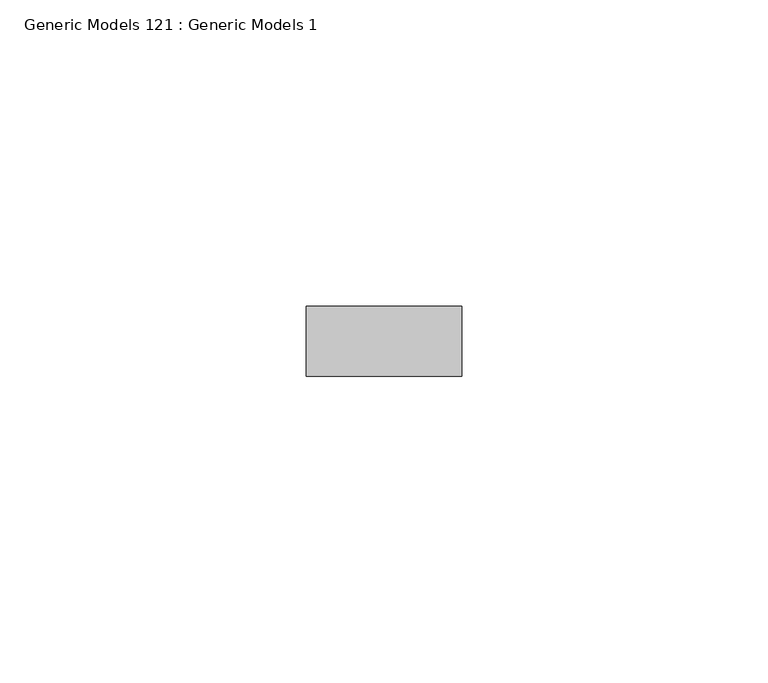
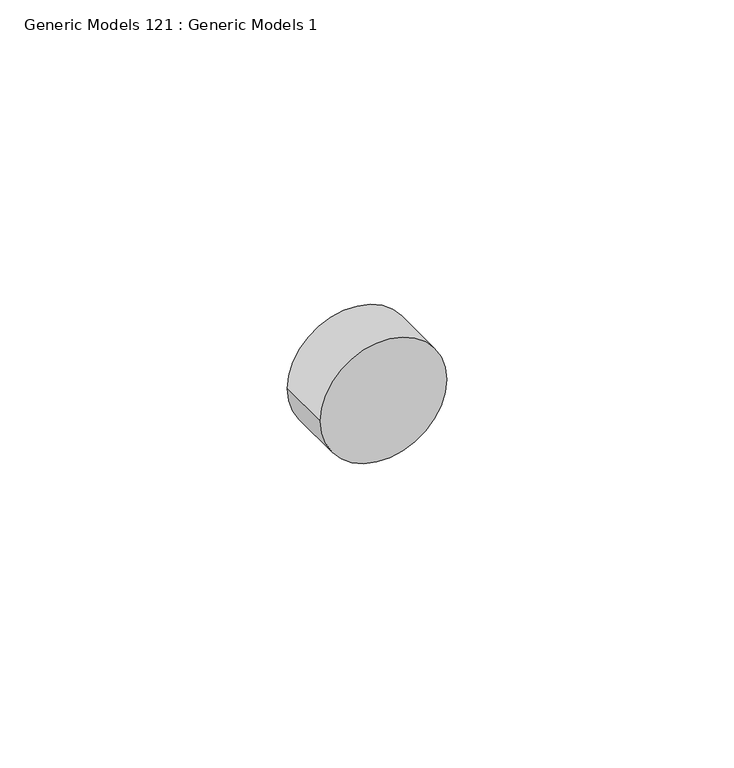
"""IFC4 building model written with IfcOpenShell, lengths in millimetres: proxy geometry, Generic Models 121 : Generic Models 1."""

from ifc_helpers import new_model, si_unit, point, frame, frame_2d, origin, place, context, project, spatial, circle_curve, trimmed, segment, composite_curve, outline, extrude, source, transform, mapped, element, save


def generic_models_121_generic_models_1_0d526897(model_context):
    return source(origin(), model_context, "Body", "SweptSolid", [
        extrude(outline(composite_curve([segment(trimmed(circle_curve(frame_2d((38203.4419837, 7407.5828124)), 12.7), [point((38203.4419837, 7394.8828124))], [point((38203.4419837, 7420.2828124))], False, "CARTESIAN"), True, "CONTINUOUS"), segment(trimmed(circle_curve(frame_2d((38203.4419837, 7407.5828124)), 12.7), [point((38203.4419837, 7420.2828124))], [point((38203.4419837, 7394.8828124))], False, "CARTESIAN"), True, "CONTINUOUS")], self_intersect=False)), frame((0.0, 1836.9202358, 0.0), z_axis=(0.0, 1.0, 0.0), x_axis=(0.0, 0.0, 1.0)), (0.0, 0.0, 1.0), 11.4464372),
    ])


if __name__ == "__main__":
    model = new_model("IFC4")
    model_context = context("Model", 3, world=origin())
    ifc_project = project(units=[si_unit("LENGTHUNIT", "METRE", prefix="MILLI")], contexts=[model_context])
    site = spatial("IfcSite", under=ifc_project)
    building = spatial("IfcBuilding", under=site)
    placement = place(None, origin())
    generic_models_121_generic_models_1_shape = generic_models_121_generic_models_1_0d526897(model_context)
    element("IfcBuildingElementProxy", 1, Name="Generic Models 121 : Generic Models 1", ObjectType="Generic Models 121 : Generic Models 1", at=placement, inside=building, context=model_context, shape_type="MappedRepresentation", body=[
        mapped(generic_models_121_generic_models_1_shape, transform((0.0, 0.0, 0.0), x_axis=(1.0, 0.0, 0.0), y_axis=(0.0, 1.0, 0.0), z_axis=(0.0, 0.0, 1.0))),
    ])
    save(model, "model.ifc")

# Revit data of these elements
# Element 1 (IfcBuildingElementProxy, "Generic Models 121 : Generic Models 1")
#   Materials on its faces: "S.S. LAG BOLT - SEE STRUCT. DWGS"
# Materials
#   "S.S. LAG BOLT - SEE STRUCT. DWGS": class "Generic", colour RGB 120 120 120, transparency 0, Cost = 0
